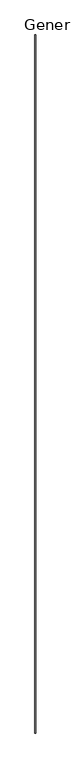
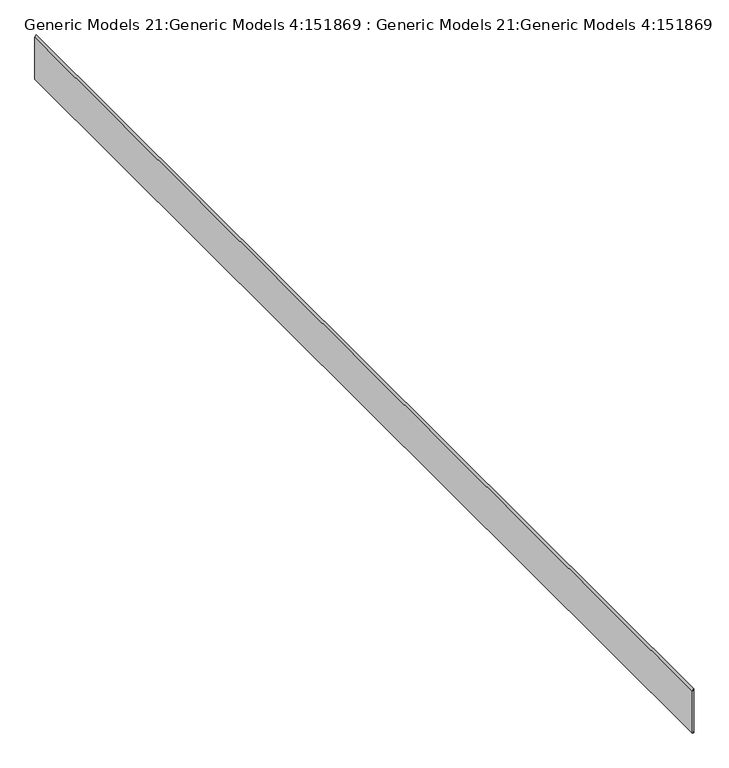
"""IFC4 building model written with IfcOpenShell, lengths in millimetres: proxy geometry, Generic Models 21:Generic Models 4:151869 : Generic Models 21:Generic Models 4:151869."""

from ifc_helpers import new_model, si_unit, frame, origin, place, context, project, spatial, polyline, outline, extrude, source, transform, mapped, element, save


def generic_models_21_generic_models_4_151869_generic_models_21_5f8a0033(model_context):
    return source(origin(), model_context, "Body", "SweptSolid", [
        extrude(outline(polyline([(3808.2495785, 8556.503213), (3770.9747574, 8537.3620887), (3046.095, 8537.3620887), (3046.095, 8555.233213), (3048.3048, 8555.233213), (3048.3048, 8554.3743722), (3068.6193787, 8554.3743722), (3068.6193787, 8555.6443722), (3049.5748, 8555.6443722), (3049.5748, 8556.503213), (3808.2495785, 8556.503213)])), frame((0.0, -6674.7974793, 0.0), z_axis=(0.0, 1.0, 0.0), x_axis=(0.0, 0.0, 1.0)), (0.0, 0.0, 1.0), 18643.6),
    ])


if __name__ == "__main__":
    model = new_model("IFC4")
    model_context = context("Model", 3, world=origin())
    ifc_project = project(units=[si_unit("LENGTHUNIT", "METRE", prefix="MILLI")], contexts=[model_context])
    site = spatial("IfcSite", under=ifc_project)
    building = spatial("IfcBuilding", under=site)
    placement = place(None, origin())
    generic_models_21_generic_models_4_151869_generic_models_21_shape = generic_models_21_generic_models_4_151869_generic_models_21_5f8a0033(model_context)
    element("IfcBuildingElementProxy", 1, Name="Generic Models 21:Generic Models 4:151869 : Generic Models 21:Generic Models 4:151869", ObjectType="Generic Models 21:Generic Models 4:151869 : Generic Models 21:Generic Models 4:151869", at=placement, inside=building, context=model_context, shape_type="MappedRepresentation", body=[
        mapped(generic_models_21_generic_models_4_151869_generic_models_21_shape, transform((0.0, 0.0, 0.0), x_axis=(1.0, 0.0, 0.0), y_axis=(0.0, 1.0, 0.0), z_axis=(0.0, 0.0, 1.0))),
    ])
    save(model, "model.ifc")

# Revit data of these elements
# Type "Generic Models 21:Generic Models 4:151869 : Generic Models 21:Generic Models 4:151869"
#   NameOverride = "Generic Models 21:Generic Models 4:151869"
#   ObjectTypeOverride = "Generic Models 21:Generic Models 4"
#   Reference = "Generic Models 4"
#   Category = "Generic Models"
#   Tag = "151869"
# Element 1 (IfcBuildingElementProxy, "Generic Models 21:Generic Models 4:151869 : Generic Models 21:Generic Models 4:151869")
#   Materials on its faces: "_7/8\" SMOOTH TROWEL EXTERIOR STUCCO (COLOR PER OWNER) 770"
# Materials
#   "_7/8\" SMOOTH TROWEL EXTERIOR STUCCO (COLOR PER OWNER) 770": class "Unassigned", colour RGB 233 233 233, transparency 0
